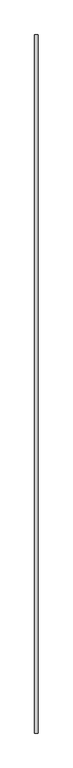
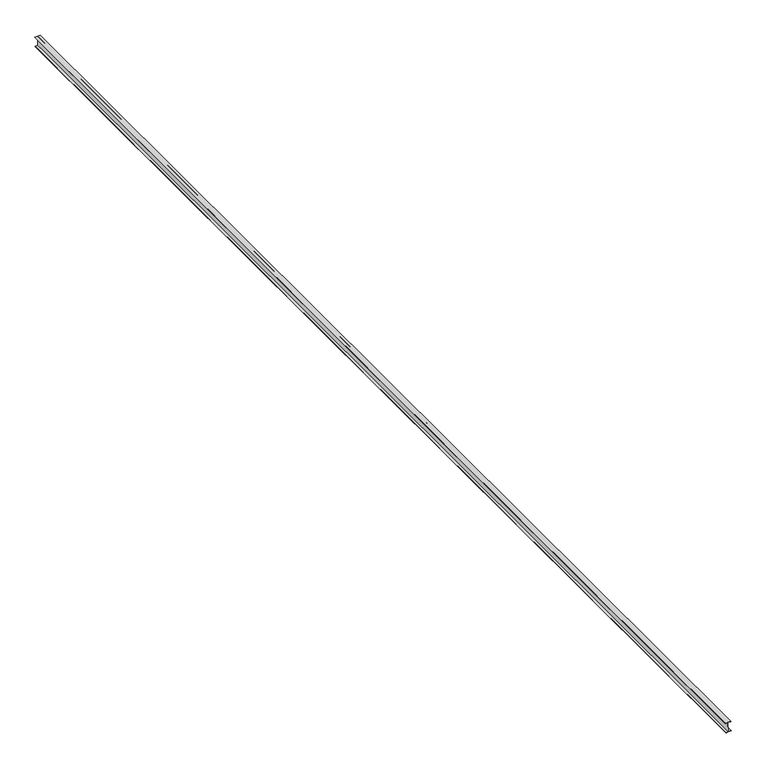
"""IFC4 building model written with IfcOpenShell, lengths in millimetres: proxy geometry, Generic Models 7:Generic Models 1:8:Generic Models 1:8 : Generic Models 7:Generic Models 1:337419:26 : Generic Models 7:Generic Models 1:8:Generic Models 1:8 : Generic Models 7:Generic Models 1:337419:315935."""

from ifc_helpers import new_model, si_unit, frame, origin, place, context, project, spatial, polyline, outline, extrude, source, transform, mapped, element, save


def generic_models_b2785e64(model_context):
    return source(origin(), model_context, "Body", "SweptSolid", [
        extrude(outline(polyline([(3670.9066459, 560594.8242278), (3674.218924, 560674.3189025), (3382.3721534, 560686.4791846), (3379.0598752, 560606.9845097), (3370.1775822, 560607.3546053), (3377.0400533, 560772.0539101), (3385.9223463, 560771.6838145), (3382.6206461, 560692.4430099), (3674.4674167, 560680.2827278), (3677.7691169, 560759.5235326), (3686.65141, 560759.1534371), (3679.7889389, 560594.4541322), (3670.9066459, 560594.8242278)])), frame((0.0, -578904.379416, 0.0), z_axis=(0.0, 1.0, 0.0), x_axis=(0.0, 0.0, 1.0)), (0.0, 0.0, 1.0), 35720.8630319),
    ])


if __name__ == "__main__":
    model = new_model("IFC4")
    model_context = context("Model", 3, world=origin())
    ifc_project = project(units=[si_unit("LENGTHUNIT", "METRE", prefix="MILLI")], contexts=[model_context])
    site = spatial("IfcSite", under=ifc_project)
    building = spatial("IfcBuilding", under=site)
    placement = place(None, origin())
    generic_models_shape = generic_models_b2785e64(model_context)
    element("IfcBuildingElementProxy", 1, Name="Generic Models 7:Generic Models 1:8:Generic Models 1:8 : Generic Models 7:Generic Models 1:337419:26 : Generic Models 7:Generic Models 1:8:Generic Models 1:8 : Generic Models 7:Generic Models 1:337419:315935", ObjectType="Generic Models 7:Generic Models 1:8:Generic Models 1:8 : Generic Models 7:Generic Models 1:337419:26 : Generic Models 7:Generic Models 1:8:Generic Models 1:8 : Generic Models 7:Generic Models 1:337419:315935", at=placement, inside=building, context=model_context, shape_type="MappedRepresentation", body=[
        mapped(generic_models_shape, transform((0.0, 0.0, 0.0), x_axis=(1.0, 0.0, 0.0), y_axis=(0.0, 1.0, 0.0), z_axis=(0.0, 0.0, 1.0))),
    ])
    save(model, "model.ifc")

# Revit data of these elements
# Type "Generic Models 7:Generic Models 1:8:Generic Models 1:8 : Generic Models 7:Generic Models 1:337419:26 : Generic Models 7:Generic Models 1:8:Generic Models 1:8 : Generic Models 7:Generic Models 1:337419:315935"
#   NameOverride = "Generic Models 7:Generic Models 1:8:Generic Models 1:8 : Generic Models 7:Generic Models 1:337419:315935"
#   ObjectTypeOverride = "Generic Models 1:8 : Generic Models 7:Generic Models 1:337419"
#   Reference = "Generic Models 1"
#   Tag = "315935"
# Element 1 (IfcBuildingElementProxy, "Generic Models 7:Generic Models 1:8:Generic Models 1:8 : Generic Models 7:Generic Models 1:337419:26 : Generic Models 7:Generic Models 1:8:Generic Models 1:8 : Generic Models 7:Generic Models 1:337419:315935")
#   Materials on its faces: "STRUCTURAL STEEL - SEE STRUCT. DWGS"
# Materials
#   "STRUCTURAL STEEL - SEE STRUCT. DWGS": class "Metal", colour RGB 189 187 185, transparency 0, Description = "Structural steel 50ksi", Cost = 0
